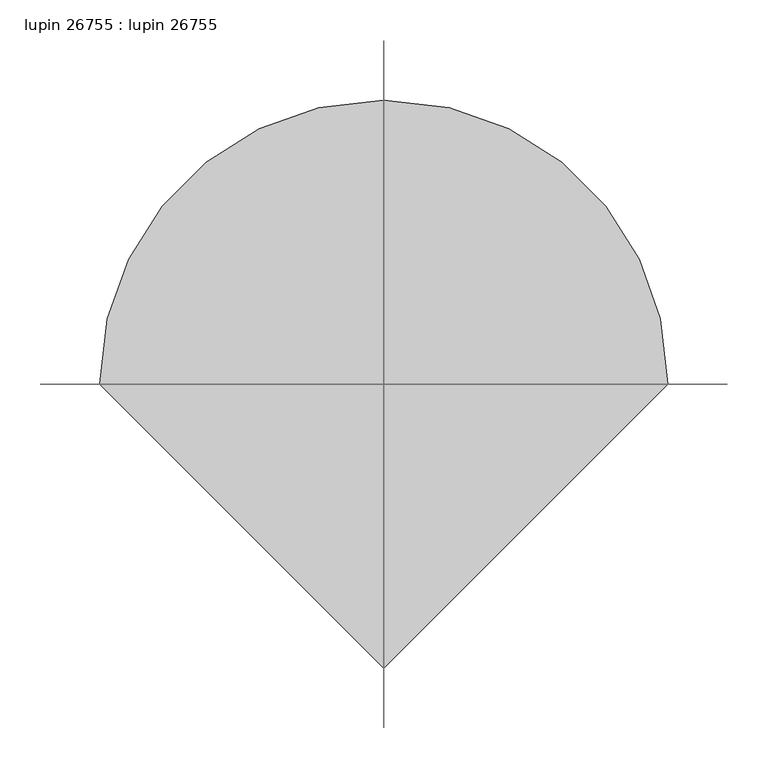
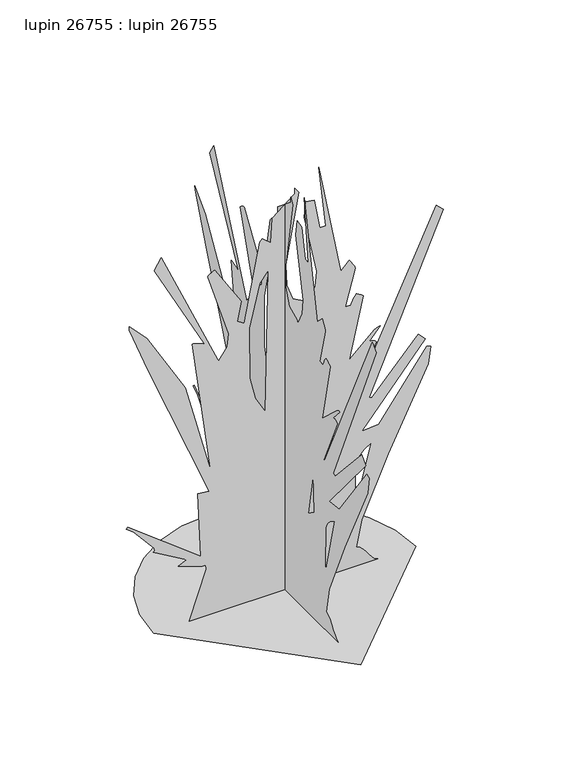
"""IFC4 building model written with IfcOpenShell, lengths in millimetres: proxy geometry, lupin 26755 : lupin 26755."""

from ifc_helpers import new_model, si_unit, origin, place, context, project, spatial, triangles, source, transform, mapped, element, save


def lupin_26755_lupin_26755_b3c85f71(model_context):
    return source(origin(), model_context, "Body", "Tessellation", [
        triangles([(-351.9469769, 0.0, 0.0), (-342.6429663, 80.6431063, 0.0), (-316.1457464, 154.7010223, 0.0), (-274.573611, 220.0515756, 0.0), (-220.0515756, 274.573611, 0.0), (-154.700768, 316.1457464, 0.0), (-80.6431063, 342.6429663, 0.0), (1.54e-05, 351.9469769, 0.0), (80.6431063, 342.6429663, 0.0), (154.7010223, 316.1457464, 0.0), (220.0515756, 274.573611, 0.0), (274.573611, 220.0515756, 0.0), (316.1457464, 154.700768, 0.0), (342.6429663, 80.6431063, 0.0), (351.9469769, -3.08e-05, 0.0), (-4.62e-05, -351.9469769, 0.0), (150.6720804, 0.0015947, 851.9910187), (173.2724542, 0.0015961, 874.5918921), (188.3394669, 0.0015947, 851.9910187), (188.5203062, 0.0015944, 847.0684994), (161.9722718, 0.0015884, 746.5202036), (177.0392664, 0.0015884, 746.5202036), (178.9694175, 0.0015886, 750.284436), (180.6039107, 0.0015889, 754.0461977), (182.1639718, 0.0015891, 757.8054159), (183.8723704, 0.0015893, 761.5671049), (185.9508409, 0.0015895, 765.3339535), (188.6214083, 0.0015898, 769.1058163), (192.1062791, 0.00159, 772.8878529), (193.2812801, 0.00159, 772.4611347), (195.5106317, 0.0015899, 771.3080074), (198.4649026, 0.0015898, 769.6264967), (201.8143893, 0.0015897, 767.6173897), (205.2296787, 0.0015896, 765.4761686), (208.3815575, 0.0015894, 763.4010046), (210.9401041, 0.0015893, 761.5874525), (173.2724542, 0.0015792, 592.0833366), (240.700733, 0.0015829, 654.2395718), (250.6943454, 0.0015832, 659.6218014), (256.1408516, 0.0015833, 659.8859568), (226.0070987, 0.0015812, 625.984683), (228.5658996, 0.0015812, 626.1598904), (231.7175241, 0.0015812, 625.7001801), (235.1327953, 0.0015812, 624.7324339), (238.4825545, 0.0015811, 623.3938528), (241.4365711, 0.001581, 621.8114639), (243.6659227, 0.0015809, 620.1197794), (244.8409236, 0.0015808, 618.4509859), (180.8060786, 0.0015725, 479.0814042), (184.572909, 0.0015725, 479.0814042), (406.8108882, 0.0016005, 949.9256659), (425.6449857, 0.0015994, 931.0915684), (226.0070987, 0.0015718, 467.7809675), (233.5407231, 0.0015716, 464.0141553), (357.8448363, 0.0015797, 599.6169611), (376.6763904, 0.0015785, 580.7828636), (207.1732737, 0.0015664, 377.3799811), (252.3745481, 0.0015666, 381.1467934), (380.4432026, 0.0015772, 558.1819902), (391.7436393, 0.001577, 554.4177215), (384.6443633, 0.0015741, 506.8385036), (278.1600926, 0.0015612, 289.3386073), (206.7572381, 0.0015515, 126.6752076), (192.1062791, 0.0015471, 53.437713), (201.6487926, 0.0015469, 49.4892894), (210.1163717, 0.0015464, 41.8553304), (217.9390592, 0.0015458, 32.010051), (225.5471159, 0.0015452, 21.427562), (233.3697852, 0.0015446, 11.5823576), (241.8373824, 0.0015442, 3.9483989), (251.3798959, 0.0015439, 1.66e-05), (-256.5091613, 0.001544, 0.4898205), (-211.4973739, 0.0015518, 132.0554297), (-212.2487088, 0.0015525, 144.4635658), (-222.2372343, 0.0015525, 143.8397394), (-286.2728424, 0.0015538, 166.4403676), (-263.6719508, 0.0015545, 177.7405681), (-354.0729735, 0.0015577, 230.4752126), (-348.9472326, 0.0015578, 232.5839138), (-351.022433, 0.0015583, 241.0403199), (-406.3257797, 0.0015621, 305.3939318), (-425.6424422, 0.0015631, 320.8777614), (-421.87563, 0.0015633, 324.6445736), (-226.0037922, 0.0015543, 173.9740102), (-233.5374348, 0.0015651, 354.7790714), (-203.4034275, 0.0015648, 351.0122592), (-366.5443417, 0.0015886, 750.3606668), (-417.7760619, 0.0015966, 882.9891266), (-418.1088178, 0.0015972, 893.4259169), (-370.8775801, 0.0015942, 843.3371864), (-268.1575782, 0.0015837, 667.2316566), (-199.6365971, 0.0015682, 407.5119355), (-248.6044294, 0.0015907, 784.1883259), (-246.3971695, 0.0015907, 784.2213181), (-242.3227634, 0.0015906, 783.3755121), (-236.9745433, 0.0015905, 781.8490065), (-230.9453692, 0.0015904, 779.8398268), (-224.8285369, 0.0015903, 777.5436733), (-219.2169245, 0.0015901, 775.1611879), (-214.7036098, 0.00159, 772.8878529), (-350.306125, 0.0016053, 1029.028759), (-331.4720638, 0.0016071, 1059.1632568), (-180.8027903, 0.0015866, 716.3881765), (-177.0359781, 0.0015864, 712.6214006), (-155.1577168, 0.0015883, 744.8692142), (-150.1099781, 0.0015904, 779.1769312), (-207.1702397, 0.0016012, 961.2260662), (-205.9949844, 0.0016013, 963.0370749), (-203.7656147, 0.0016014, 965.1147823), (-194.0468402, 0.0016018, 970.9440777), (-190.8949614, 0.0016019, 972.0972776), (-188.3364148, 0.0016019, 972.5265392), (-116.7679544, 0.0015952, 859.5246431), (-128.0681458, 0.001592, 806.7891993), (-109.2343208, 0.0015913, 795.4887989), (-67.8001221, 0.0016041, 1010.1946615), (-60.2664931, 0.0016046, 1017.728286), (-37.6658604, 0.0016035, 998.8941885), (-33.8993003, 0.0016075, 1066.6968813), (26.3689732, 0.0016104, 1115.6629332), (26.3689732, 0.0016113, 1130.7301821), (37.6691624, 0.0016104, 1115.6629332), (2.9836067, 0.0015988, 921.19319), (5.2254839, 0.0015953, 862.2830503), (21.4607608, 0.0015927, 818.4376162), (56.5029828, 0.0015916, 799.2555748), (60.269795, 0.0015911, 791.7219503), (81.2288264, 0.0015936, 833.4109028), (86.0914021, 0.0015961, 874.8052511), (51.7460784, 0.0016059, 1039.955781), (56.5029828, 0.0016084, 1081.7615868), (79.10362, 0.0016082, 1077.9948109), (94.1706237, 0.0016032, 995.1274126), (109.237373, 0.0016032, 995.1274126), (90.4038023, 0.0016136, 1168.3983044), (-67.325905, 0.0015972, 893.4183592), (-96.1172708, 0.0015902, 776.6851501), (-94.9783414, 0.0015817, 633.9373953), (-79.6923831, 0.001578, 571.2782112), (-52.7331184, 0.0015752, 524.2831873), (-45.1994894, 0.001599, 923.5579439), (109.237373, 0.0015608, 283.2096027), (135.6048224, 0.0015619, 302.0436639), (131.8382554, 0.0015682, 407.5119355), (211.912919, 0.0015632, 322.7039944), (198.2078507, 0.0015623, 307.9059877), (189.9752137, 0.0015612, 290.5146256), (188.3394669, 0.0015547, 181.5073803), (192.1062791, 0.0015545, 177.7405681), (232.2618404, 0.0015639, 335.5792259), (0.0016106, -150.6687739, 851.9910187), (0.0016109, -173.269402, 874.5918921), (0.00161, -188.3364148, 851.9910187), (0.0016099, -188.5169997, 847.0684994), (0.0016073, -161.9689653, 746.5202036), (0.001607, -177.0362324, 746.5202036), (0.0016071, -178.9663653, 750.284436), (0.0016072, -180.6006042, 754.0461977), (0.0016073, -182.1609196, 757.8054159), (0.0016074, -183.8693182, 761.5671049), (0.0016075, -185.9478069, 765.3339535), (0.0016076, -188.6183561, 769.1058163), (0.0016076, -192.103227, 772.8878529), (0.0016076, -193.2782279, 772.4611347), (0.0016075, -195.5075795, 771.3080074), (0.0016074, -198.4615962, 769.6264967), (0.0016073, -201.8113554, 767.6173897), (0.0016072, -205.2266265, 765.4761686), (0.0016071, -208.378251, 763.4010046), (0.001607, -210.937052, 761.5874525), (0.0016025, -173.269402, 592.0833366), (0.0016033, -240.6974266, 654.2395718), (0.0016034, -250.6910389, 659.6218014), (0.0016033, -256.1383082, 659.8859568), (0.0016027, -226.0040465, 625.984683), (0.0016027, -228.5625931, 626.1598904), (0.0016026, -231.7142176, 625.7001801), (0.0016026, -235.1297431, 624.7324339), (0.0016025, -238.479248, 623.3938528), (0.0016024, -241.4332646, 621.8114639), (0.0016023, -243.6626162, 620.1197794), (0.0016022, -244.8378715, 618.4509859), (0.001599, -180.8027903, 479.0814042), (0.001599, -184.5696025, 479.0814042), (0.0016097, -406.8083447, 949.9256659), (0.0016088, -425.6424422, 931.0915684), (0.001598, -226.0040465, 467.7809675), (0.0015978, -233.5374348, 464.0141553), (0.0016, -357.8397858, 599.6169611), (0.0015991, -376.6738469, 580.7828636), (0.0015956, -207.1702397, 377.3799811), (0.001595, -252.3712416, 381.1467934), (0.0015984, -380.4406591, 558.1845337), (0.0015981, -391.7410958, 554.4177215), (0.0015968, -384.6418199, 506.8385036), (0.0015919, -278.1575492, 289.3386073), (0.0015881, -206.7539316, 126.6752076), (0.0015862, -192.103227, 53.437713), (0.0015859, -201.6454861, 49.4892894), (0.0015856, -210.1130652, 41.8553304), (0.0015851, -217.936007, 32.010051), (0.0015847, -225.5438094, 21.427587), (0.0015843, -233.3664787, 11.5823837), (0.001584, -241.8343303, 3.9483989), (0.0015837, -251.3765894, 2.41e-05), (0.0015913, 256.51423, 0.4898434), (0.0015945, 211.5006804, 132.0554297), (0.0015949, 212.2519971, 144.4635658), (0.001595, 222.2402864, 143.8397394), (0.0015967, 286.2753676, 166.4403676), (0.0015967, 263.6744943, 177.7405681), (0.0015996, 354.0780241, 230.4752126), (0.0015996, 348.9497761, 232.5839138), (0.0015999, 351.0249764, 241.0403199), (0.0016026, 406.3308303, 305.3939318), (0.0016033, 425.6449857, 320.8777614), (0.0016034, 421.8781734, 324.6445736), (0.001596, 226.0070987, 173.9740102), (0.0016015, 233.5404688, 354.7790714), (0.0016009, 203.4064615, 351.0122592), (0.0016153, 366.5468851, 750.3606668), (0.00162, 417.7786054, 882.9891266), (0.0016203, 418.1113612, 893.4259169), (0.0016181, 370.8801235, 843.3371864), (0.0016113, 268.1626651, 667.2316566), (0.0016026, 199.6396492, 407.5119355), (0.0016145, 248.6077359, 784.1883259), (0.0016145, 246.4002216, 784.2213181), (0.0016144, 242.3260699, 783.3755121), (0.0016143, 236.9775955, 781.8490065), (0.0016141, 230.9484032, 779.8398268), (0.001614, 224.8318434, 777.5436733), (0.0016138, 219.2199766, 775.1611879), (0.0016137, 214.7069163, 772.8878529), (0.0016233, 350.3112119, 1029.028759), (0.0016239, 331.4771507, 1059.1632568), (0.0016115, 180.8060786, 716.3881765), (0.0016113, 177.0392664, 712.6214006), (0.001612, 155.1607508, 744.8692142), (0.0016129, 150.1132755, 779.1769312), (0.0016192, 207.1732737, 961.2260662), (0.0016192, 205.9982728, 963.0396183), (0.0016192, 203.7689212, 965.1147823), (0.0016193, 194.0498742, 970.9466211), (0.0016193, 190.8979953, 972.0998211), (0.0016192, 188.3394669, 972.5265392), (0.0016148, 116.7709974, 859.5246431), (0.0016134, 128.0714432, 806.7891993), (0.0016128, 109.2376273, 795.4887989), (0.0016186, 67.8031697, 1010.1946615), (0.0016187, 60.269795, 1017.728286), (0.0016178, 37.6691624, 998.8941885), (0.0016197, 33.9023479, 1066.6968813), (0.0016203, -26.3656713, 1115.6629332), (0.0016207, -26.3656713, 1130.7301821), (0.0016201, -37.6661148, 1115.6629332), (0.0016148, -2.9804319, 921.19319), (0.0016131, -5.2223085, 862.2830503), (0.0016115, -21.4575588, 818.4376162), (0.0016104, -56.4999352, 799.2555748), (0.0016101, -60.2664931, 791.7219503), (0.0016111, -81.225529, 833.4109028), (0.0016122, -86.0883499, 874.8052511), (0.0016177, -51.7430263, 1039.955781), (0.0016188, -56.4999352, 1081.7615868), (0.0016184, -79.1003135, 1077.9948109), (0.0016157, -94.1673172, 995.1274126), (0.0016155, -109.2340665, 995.1274126), (0.0016209, -90.4007593, 1168.3983044), (0.0016151, 67.329207, 893.4183592), (0.001612, 96.120323, 776.6851501), (0.0016077, 94.9816388, 633.9373953), (0.0016057, 79.6956896, 571.2782112), (0.0016039, 52.736166, 524.2831873), (0.0016156, 45.202537, 923.5579439), (0.0015943, -109.2340665, 283.2096027), (0.0015944, -135.6017703, 302.0436639), (0.0015976, -131.834958, 407.5119355), (0.0015939, -211.9098669, 322.7039944), (0.0015937, -198.2045624, 307.9059877), (0.0015933, -189.9719254, 290.5146256), (0.00159, -188.3364148, 181.5073803), (0.0015899, -192.103227, 177.7405681), (0.001594, -232.2587883, 335.5792259)], [[16, 15, 1], [15, 14, 1], [1, 14, 2], [14, 13, 2], [2, 13, 3], [3, 13, 4], [13, 12, 4], [12, 11, 4], [4, 11, 5], [5, 11, 6], [6, 11, 7], [7, 11, 8], [8, 11, 9], [9, 11, 10], [142, 144, 18], [135, 134, 17], [71, 70, 72], [121, 120, 122], [18, 17, 142], [17, 140, 142], [89, 88, 90], [70, 69, 72], [40, 39, 41], [39, 38, 41], [38, 37, 41], [76, 75, 77], [78, 77, 79], [69, 68, 72], [102, 101, 103], [101, 100, 103], [68, 67, 72], [67, 66, 72], [66, 65, 72], [65, 64, 72], [148, 147, 143], [51, 50, 52], [52, 50, 53], [120, 119, 122], [119, 118, 122], [143, 142, 148], [85, 84, 86], [72, 64, 73], [93, 92, 94], [94, 92, 95], [95, 92, 96], [96, 92, 97], [97, 92, 98], [98, 92, 99], [99, 92, 100], [100, 92, 103], [103, 92, 104], [82, 81, 83], [83, 81, 84], [81, 80, 84], [80, 79, 84], [79, 77, 84], [77, 75, 84], [131, 130, 132], [132, 130, 133], [55, 54, 56], [56, 54, 57], [64, 63, 73], [88, 87, 90], [90, 87, 91], [91, 87, 92], [87, 86, 92], [75, 74, 84], [73, 63, 74], [117, 116, 118], [116, 115, 118], [122, 118, 123], [54, 53, 57], [53, 50, 57], [60, 59, 61], [59, 58, 61], [61, 58, 62], [58, 57, 62], [50, 49, 57], [147, 146, 143], [143, 146, 144], [146, 145, 144], [145, 150, 144], [134, 133, 17], [133, 130, 17], [130, 129, 17], [129, 128, 17], [17, 128, 140], [128, 127, 140], [29, 28, 30], [36, 35, 37], [35, 34, 37], [34, 33, 37], [33, 32, 37], [32, 31, 37], [31, 30, 37], [30, 28, 37], [28, 27, 37], [27, 26, 37], [26, 25, 37], [25, 24, 37], [24, 23, 37], [23, 22, 37], [22, 21, 37], [112, 111, 113], [111, 110, 113], [110, 109, 113], [109, 108, 113], [108, 107, 113], [113, 107, 114], [107, 106, 114], [74, 63, 84], [84, 63, 86], [86, 63, 92], [48, 47, 49], [47, 46, 49], [46, 45, 49], [45, 44, 49], [44, 43, 49], [43, 42, 49], [42, 41, 49], [41, 37, 49], [92, 63, 104], [106, 105, 114], [114, 105, 115], [127, 126, 140], [126, 125, 140], [140, 125, 141], [125, 124, 141], [124, 123, 141], [123, 118, 141], [141, 118, 136], [118, 115, 136], [136, 115, 137], [115, 105, 137], [105, 104, 137], [137, 104, 138], [138, 104, 139], [19, 18, 20], [20, 18, 21], [18, 144, 21], [21, 144, 37], [37, 144, 49], [49, 144, 57], [144, 150, 57], [57, 150, 62], [150, 149, 62], [62, 149, 63], [149, 148, 63], [148, 142, 63], [139, 104, 140], [104, 63, 140], [140, 63, 142], [276, 278, 152], [269, 268, 151], [205, 204, 206], [255, 254, 256], [152, 151, 276], [151, 274, 276], [223, 222, 224], [204, 203, 206], [174, 173, 175], [173, 172, 175], [172, 171, 175], [210, 209, 211], [212, 211, 213], [203, 202, 206], [236, 235, 237], [235, 234, 237], [202, 201, 206], [201, 200, 206], [200, 199, 206], [199, 198, 206], [282, 281, 277], [185, 184, 186], [186, 184, 187], [254, 253, 256], [253, 252, 256], [277, 276, 282], [219, 218, 220], [206, 198, 207], [227, 226, 228], [228, 226, 229], [229, 226, 230], [230, 226, 231], [231, 226, 232], [232, 226, 233], [233, 226, 234], [234, 226, 237], [237, 226, 238], [216, 215, 217], [217, 215, 218], [215, 214, 218], [214, 213, 218], [213, 211, 218], [211, 209, 218], [265, 264, 266], [266, 264, 267], [189, 188, 190], [190, 188, 191], [198, 197, 207], [222, 221, 224], [224, 221, 225], [225, 221, 226], [221, 220, 226], [209, 208, 218], [207, 197, 208], [251, 250, 252], [250, 249, 252], [256, 252, 257], [188, 187, 191], [187, 184, 191], [194, 193, 195], [193, 192, 195], [195, 192, 196], [192, 191, 196], [184, 183, 191], [281, 280, 277], [277, 280, 278], [280, 279, 278], [279, 284, 278], [268, 267, 151], [267, 264, 151], [264, 263, 151], [263, 262, 151], [151, 262, 274], [262, 261, 274], [163, 162, 164], [170, 169, 171], [169, 168, 171], [168, 167, 171], [167, 166, 171], [166, 165, 171], [165, 164, 171], [164, 162, 171], [162, 161, 171], [161, 160, 171], [160, 159, 171], [159, 158, 171], [158, 157, 171], [157, 156, 171], [156, 155, 171], [246, 245, 247], [245, 244, 247], [244, 243, 247], [243, 242, 247], [242, 241, 247], [247, 241, 248], [241, 240, 248], [208, 197, 218], [218, 197, 220], [220, 197, 226], [182, 181, 183], [181, 180, 183], [180, 179, 183], [179, 178, 183], [178, 177, 183], [177, 176, 183], [176, 175, 183], [175, 171, 183], [226, 197, 238], [240, 239, 248], [248, 239, 249], [261, 260, 274], [260, 259, 274], [274, 259, 275], [259, 258, 275], [258, 257, 275], [257, 252, 275], [275, 252, 270], [252, 249, 270], [270, 249, 271], [249, 239, 271], [239, 238, 271], [271, 238, 272], [272, 238, 273], [153, 152, 154], [154, 152, 155], [152, 278, 155], [155, 278, 171], [171, 278, 183], [183, 278, 191], [278, 284, 191], [191, 284, 196], [284, 283, 196], [196, 283, 197], [283, 282, 197], [282, 276, 197], [273, 238, 274], [238, 197, 274], [274, 197, 276]], closed=False),
    ])


if __name__ == "__main__":
    model = new_model("IFC4")
    model_context = context("Model", 3, world=origin())
    ifc_project = project(units=[si_unit("LENGTHUNIT", "METRE", prefix="MILLI")], contexts=[model_context])
    site = spatial("IfcSite", under=ifc_project)
    building = spatial("IfcBuilding", under=site)
    placement = place(None, origin())
    lupin_26755_lupin_26755_shape = lupin_26755_lupin_26755_b3c85f71(model_context)
    element("IfcBuildingElementProxy", 1, Name="lupin 26755 : lupin 26755", ObjectType="lupin 26755 : lupin 26755", at=placement, inside=building, context=model_context, shape_type="MappedRepresentation", body=[
        mapped(lupin_26755_lupin_26755_shape, transform((0.0, 0.0, 0.0), x_axis=(1.0, 0.0, 0.0), y_axis=(0.0, 1.0, 0.0), z_axis=(0.0, 0.0, 1.0))),
    ])
    save(model, "model.ifc")

# Revit data of these elements
# Type "lupin 26755 : lupin 26755"
#   built-in parameter 1005195 = "RPC-16-G2M4-C67X-C72M-U000-ST1L-LVER-AU"
#   Height = 0
